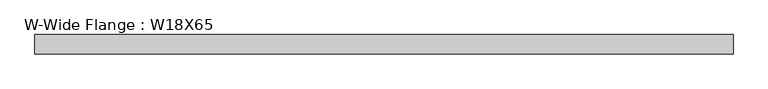
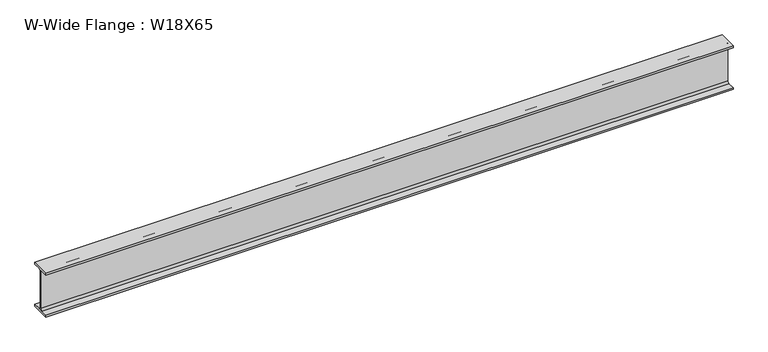
"""IFC4 building model written with IfcOpenShell, lengths in millimetres: beam geometry, W-Wide Flange : W18X65."""

from ifc_helpers import new_model, si_unit, point, frame, frame_2d, origin, place, context, project, spatial, polyline, circle_curve, trimmed, segment, composite_curve, outline, extrude, source, transform, mapped, element, save


def w_wide_flange_w18x65_d5707ef7(model_context):
    return source(origin(), model_context, "Body", "SweptSolid", [
        extrude(outline(composite_curve([segment(polyline([(96.393, -214.63), (96.393, -233.68), (-96.393, -233.68), (-96.393, -214.63), (-23.1775, -214.63)]), True, "CONTINUOUS"), segment(trimmed(circle_curve(frame_2d((-23.1775, -197.1675)), 17.4625), [point((-23.1775, -214.63))], [point((-5.715, -197.1675))], True, "CARTESIAN"), True, "CONTINUOUS"), segment(polyline([(-5.715, -197.1675), (-5.715, 197.1675)]), True, "CONTINUOUS"), segment(trimmed(circle_curve(frame_2d((-23.1775, 197.1675)), 17.4625), [point((-5.715, 197.1675))], [point((-23.1775, 214.63))], True, "CARTESIAN"), True, "CONTINUOUS"), segment(polyline([(-23.1775, 214.63), (-96.393, 214.63), (-96.393, 233.68), (96.393, 233.68), (96.393, 214.63), (23.1775, 214.63)]), True, "CONTINUOUS"), segment(trimmed(circle_curve(frame_2d((23.1775, 197.1675)), 17.4625), [point((23.1775, 214.63))], [point((5.715, 197.1675))], True, "CARTESIAN"), True, "CONTINUOUS"), segment(polyline([(5.715, 197.1675), (5.715, -197.1675)]), True, "CONTINUOUS"), segment(trimmed(circle_curve(frame_2d((23.1775, -197.1675)), 17.4625), [point((5.715, -197.1675))], [point((23.1775, -214.63))], True, "CARTESIAN"), True, "CONTINUOUS"), segment(polyline([(23.1775, -214.63), (96.393, -214.63)]), True, "CONTINUOUS")], self_intersect=False)), frame((-3479.8, 0.0, 0.0), z_axis=(1.0, 0.0, 0.0), x_axis=(0.0, 1.0, 0.0)), (0.0, 0.0, 1.0), 6959.6),
    ])


if __name__ == "__main__":
    model = new_model("IFC4")
    model_context = context("Model", 3, world=origin())
    ifc_project = project(units=[si_unit("LENGTHUNIT", "METRE", prefix="MILLI")], contexts=[model_context])
    site = spatial("IfcSite", under=ifc_project)
    building = spatial("IfcBuilding", under=site)
    placement = place(None, origin())
    w_wide_flange_w18x65_shape = w_wide_flange_w18x65_d5707ef7(model_context)
    element("IfcBeam", 1, ObjectType="W-Wide Flange : W18X65", at=placement, inside=building, context=model_context, shape_type="MappedRepresentation", body=[
        mapped(w_wide_flange_w18x65_shape, transform((0.0, 0.0, 0.0), x_axis=(1.0, 0.0, 0.0), y_axis=(0.0, 1.0, 0.0), z_axis=(0.0, 0.0, 1.0))),
    ])
    save(model, "model.ifc")

# Revit data of these elements
# Type "W-Wide Flange : W18X65"
#   Assembly Code = "B10"
#   W = 65
#   Length [instance default] = 5' - 0"
#   bf = 0' - 7.59"
#   d = 1' - 6.4"
#   k = 0' - 1 7/16"
#   k2 = 0' - 0 11/16"
#   tf = 0' - 0 3/4"
#   tw = 0' - 0.45"
#   A = 0.132639 SF
#   Structural Material [instance default] = Steel ASTM A992
# Element 1 (IfcBeam, "W-Wide Flange : W18X65")
#   Materials on its faces: "Steel ASTM A992"
# Materials
#   "Steel ASTM A992": class "Metal", colour RGB 199 199 199, transparency 0, Description = "Structural steel 50ksi", Cost = 0
